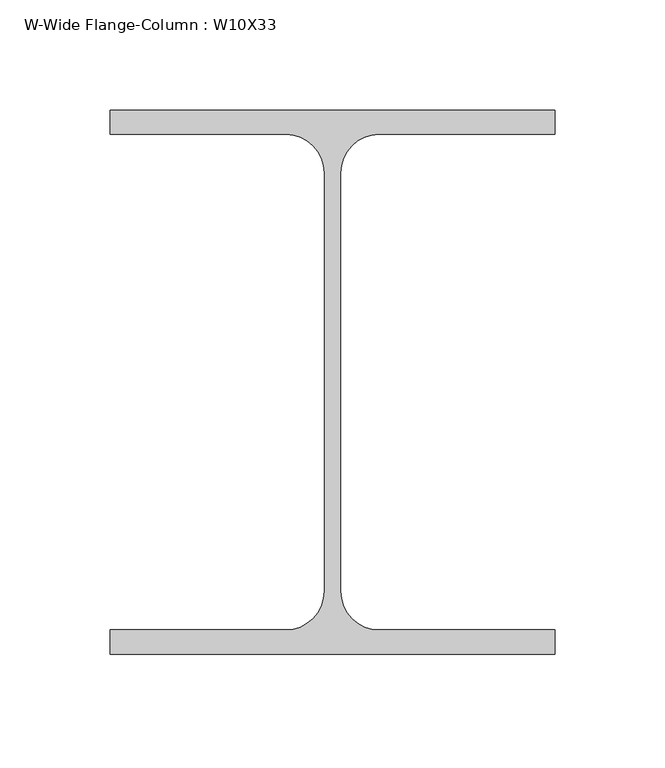
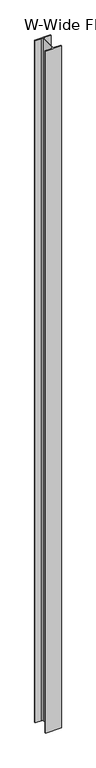
"""IFC4 building model written with IfcOpenShell, lengths in millimetres: column geometry, W-Wide Flange-Column : W10X33."""

from ifc_helpers import new_model, si_unit, point, frame, frame_2d, origin, place, context, project, spatial, polyline, circle_curve, trimmed, segment, composite_curve, outline, extrude, source, transform, mapped, element, save


def w_wide_flange_column_w10x33_efc84e3e(model_context):
    return source(origin(), model_context, "Body", "SweptSolid", [
        extrude(outline(composite_curve([segment(polyline([(101.092, 123.571), (101.092, 112.522), (21.209, 112.522)]), True, "CONTINUOUS"), segment(trimmed(circle_curve(frame_2d((21.209, 94.996)), 17.526), [point((21.209, 112.522))], [point((3.683, 94.996))], True, "CARTESIAN"), True, "CONTINUOUS"), segment(polyline([(3.683, 94.996), (3.683, -94.996)]), True, "CONTINUOUS"), segment(trimmed(circle_curve(frame_2d((21.209, -94.996)), 17.526), [point((3.683, -94.996))], [point((21.209, -112.522))], True, "CARTESIAN"), True, "CONTINUOUS"), segment(polyline([(21.209, -112.522), (101.092, -112.522), (101.092, -123.571), (-101.092, -123.571), (-101.092, -112.522), (-21.209, -112.522)]), True, "CONTINUOUS"), segment(trimmed(circle_curve(frame_2d((-21.209, -94.996)), 17.526), [point((-21.209, -112.522))], [point((-3.683, -94.996))], True, "CARTESIAN"), True, "CONTINUOUS"), segment(polyline([(-3.683, -94.996), (-3.683, 94.996)]), True, "CONTINUOUS"), segment(trimmed(circle_curve(frame_2d((-21.209, 94.996)), 17.526), [point((-3.683, 94.996))], [point((-21.209, 112.522))], True, "CARTESIAN"), True, "CONTINUOUS"), segment(polyline([(-21.209, 112.522), (-101.092, 112.522), (-101.092, 123.571), (101.092, 123.571)]), True, "CONTINUOUS")], self_intersect=False)), frame((0.0, 0.0, 12566.65), z_axis=(0.0, 0.0, 1.0), x_axis=(1.0, 0.0, 0.0)), (0.0, 0.0, 1.0), 9328.15),
    ])


if __name__ == "__main__":
    model = new_model("IFC4")
    model_context = context("Model", 3, world=origin())
    ifc_project = project(units=[si_unit("LENGTHUNIT", "METRE", prefix="MILLI")], contexts=[model_context])
    site = spatial("IfcSite", under=ifc_project)
    building = spatial("IfcBuilding", under=site)
    placement = place(None, origin())
    w_wide_flange_column_w10x33_shape = w_wide_flange_column_w10x33_efc84e3e(model_context)
    element("IfcColumn", 1, ObjectType="W-Wide Flange-Column : W10X33", at=placement, inside=building, context=model_context, shape_type="MappedRepresentation", body=[
        mapped(w_wide_flange_column_w10x33_shape, transform((0.0, 0.0, 0.0), x_axis=(1.0, 0.0, 0.0), y_axis=(0.0, 1.0, 0.0), z_axis=(0.0, 0.0, 1.0))),
    ])
    save(model, "model.ifc")

# Revit data of these elements
# Type "W-Wide Flange-Column : W10X33"
#   Assembly Code = "B10"
#   W = 33
#   bf = 0' - 7.96"
#   d = 0' - 9.73"
#   k = 0' - 1 1/8"
#   kr = 0' - 0.69"
#   tf = 0' - 0.435"
#   tw = 0' - 0.29"
#   A = 0.0674306 SF
#   Structural Material [instance default] = Steel ASTM A992
# Element 1 (IfcColumn, "W-Wide Flange-Column : W10X33")
#   Materials on its faces: "Steel ASTM A992"
# Materials
#   "Steel ASTM A992": class "Metal", colour RGB 199 199 199, transparency 0, Description = "Structural steel 50ksi", Cost = 0
